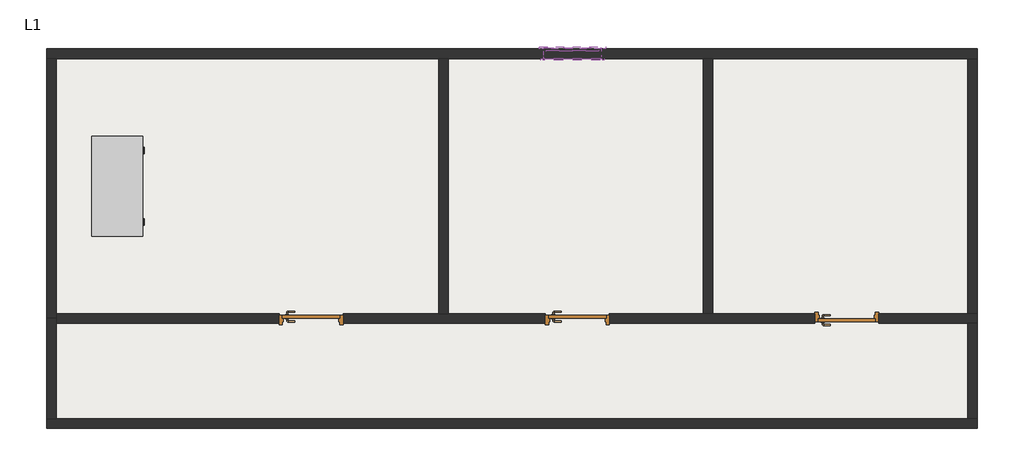
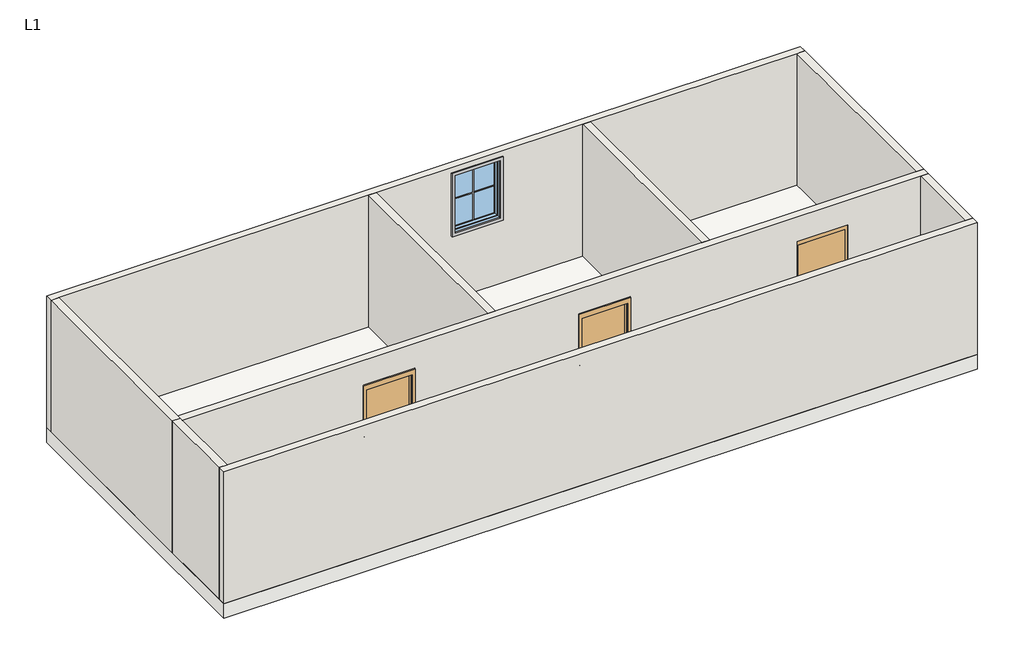
# One storey: 9 walls, 3 doors, 3 proxies, 1 furniture element, 1 slab, 1 window.
# Revit data of these elements (continued)
# Type "M_Muntin Pattern_2x2 : M_Muntin Pattern_2x2" (continued)
#   Width [instance default] = 1200 mm
#   Thickness = 12.7 mm
#   Height [instance default] = 1200 mm
#   Distance = 19.05 mm
#   Interior Material [instance default] = none
#   Exterior Material [instance default] = none
#   Default Elevation = 0
# Type "M_Trim-Window-Exterior-Flat : with Sill"
#   Trim Width = 60 mm
#   Trim Thickness_Picture Frame = 30 mm
#   Trim Thickness_with Sill = 19.05 mm
#   Sill Thickness = 30 mm
#   Opening Width [instance default] = 600 mm
#   Opening Height [instance default] = 900 mm
#   Default Elevation = 1200 mm
#   Sill = yes
#   Picture Frame = no
#   Trim Material [instance default] = none
# Type "M_Trim-Window-Interior-Flat : Picture Frame"
#   Trim Thickness_Picture Frame = 30 mm
#   Trim Width = 60 mm
#   Trim Thickness_with Sill = 20 mm
#   Sill Thickness = 30 mm
#   Opening Width [instance default] = 600 mm
#   Opening Height [instance default] = 900 mm
#   Default Elevation = 1200 mm
#   Sill = no
#   Picture Frame = yes
#   Trim Material [instance default] = none
# Type "M_Door-Passage-Single-Flush : 900 x 2100mm"
#   Type Mark = "38"
#   Analytic Construction = "Wooden"
#   Thickness = 45 mm
#   Thermal Resistance (R) = 0.455703 (m²·K)/W
#   Swing Angle [instance default] = 90.00°
#   Strike Height = 1000 mm
#   Rough Width [instance default] = 1000 mm
#   Rough Height [instance default] = 2200 mm
#   MF Opening Height [instance default] = 100 mm
#   MF Opening Width [instance default] = 100 mm
#   Inset Calculate [instance default] = 105 mm
#   Masonry Inset [instance default] = 25 mm
#   Height = 2100 mm
#   Width = 900 mm
#   Heat Transfer Coefficient (U) = 2.19465 W/(m²·K)
#   Masonry Frame Depth = 150 mm
#   Masonry Frame [instance default] = yes
#   Function = 1
#   Dry Wall Frame [instance default] = no
#   Panel Material = Wood - Birch
#   Frame Material = Metal - Paint Finish - Grey
#   Door Handle Material = Aluminum
#   Visual Light Transmittance = 0
#   Solar Heat Gain Coefficient = 0
#   Wall Closure = (empty or 0)
# Type "M_Desk : 1525 x 762mm Student"
#   Depth = 762 mm
#   Height = 762 mm
#   Leg Height = 152 mm
#   Width = 1525 mm
#   Body Material = Laminate, Ivory, Matte
#   Handle/Leg Material = Steel, Chrome Plated
#   Top Material = Cherry
#   Default Elevation = 0
# Type "Generic 300mm"
#   Description = "Generic Floor (Material By Category), 300mm thick"
#   Function = 0
#   Layers, outside or top first: 300 mm no material (function 1)
# Type "Generic - 150mm"
#   Description = "Generic Wall (Material By Category), 150mm thick"
#   Type Mark = "G04"
#   Layers, outside or top first: 150 mm no material (function 1)
# Type "M_Window-Fixed : 900 x 1200mm"
#   Type Mark = "36"
#   Fire Rating = "0.5h"
#   Analytic Construction = "Double glazing - domestic"
#   Window Inset [instance default] = 0 mm
#   Wall Thickness [instance default] = 150 mm
#   Visual Light Transmittance = 0.81
#   Thermal Resistance (R) = 0.319569 (m²·K)/W
#   Solar Heat Gain Coefficient = 0.76
#   Rough Width = 915 mm
#   Rough Height = 1215 mm
#   Interior Wall Closure [instance default] = 54.75 mm
#   Height = 1200 mm
#   Heat Transfer Coefficient (U) = 3.12929 W/(m²·K)
#   Frame Extension [instance default] = 6.35 mm
#   Exterior Wall Closure [instance default] = 31.75 mm
#   Extension Jamb [instance default] = 54.75 mm
#   Default Sill Height = 900 mm
#   Width = 900 mm
#   Muntin Visibility = yes
#   Interior Trim Visibility [instance default] = yes
#   Exterior Trim Visibility [instance default] = yes
#   Extension Jamb Visibility [instance default] = yes
#   Muntin Pattern = M_Muntin Pattern_2x2 : M_Muntin Pattern_2x2
#   Interior Trim Material = Wood - Stained
#   Interior Trim = M_Trim-Window-Interior-Flat : Picture Frame
#   Interior Frame Material = Wood - Stained
#   Glass Panel Material = Glass
#   Exterior Trim Material = Clad - White
#   Exterior Trim = M_Trim-Window-Exterior-Flat : with Sill
#   Exterior Frame Material = Clad - White
#   Wall Closure = (empty or 0)
# Element 1 (IfcBuildingElementProxy, "M_Muntin Pattern_2x2 : M_Muntin Pattern_2x2")
#   Width = 823.8 mm
#   Height = 1123.8 mm
#   Interior Material = Wood - Stained
#   Exterior Material = Clad - White
#   Phase Created = New Construction
#   Materials on its faces: "Clad - White", "Wood - Stained"
# Element 2 (IfcBuildingElementProxy, "M_Trim-Window-Exterior-Flat : with Sill")
#   Opening Width = 900 mm
#   Opening Height = 1200 mm
#   Trim Material = Clad - White
#   Phase Created = New Construction
#   Materials on its faces: "Clad - White"
# Element 3 (IfcBuildingElementProxy, "M_Trim-Window-Interior-Flat : Picture Frame")
#   Opening Width = 900 mm
#   Opening Height = 1200 mm
#   Trim Material = Wood - Stained
#   Phase Created = New Construction
#   Materials on its faces: "Wood - Stained"
# Elements 4, 5, 6 (IfcDoor, "M_Door-Passage-Single-Flush : 900 x 2100mm")
#   Swing Angle = 90.00°
#   Rough Width = 1000 mm
#   Rough Height = 2200 mm
#   Masonry Inset = 25 mm
#   MF Opening Width = 100 mm
#   MF Opening Height = 100 mm
#   Inset Calculate = 105 mm
#   Masonry Frame = yes
#   Dry Wall Frame = no
#   Phase Created = New Construction
#   Materials on its faces: "Aluminum", "Metal - Paint Finish - Grey", "Wood - Birch"
# Element 7 (IfcFurniture, "M_Desk : 1525 x 762mm Student")
#   Phase Created = New Construction
#   Materials on its faces: "Steel, Chrome Plated", "Laminate, Ivory, Matte", "Cherry"
# Element 8 (IfcSlab, "Generic 300mm")
#   Height Offset From Level = 0 mm
#   Phase Created = New Construction
#   Materials on its faces: "Default Floor"
# Elements 9, 10, 11, 12, 13, 14, 15, 17 (IfcWall, "Generic - 150mm")
#   Top Offset = 0 mm
#   Base Offset = 0 mm
#   Unconnected Height = 2700 mm
#   wall height = 2700 mm
#   Phase Created = New Construction
#   Base Constraint = L1
#   Materials on its faces: "Default Wall"
# Element 16 (IfcWall, "Generic - 150mm")
#   Top Offset = 0 mm
#   Base Offset = 0 mm
#   wall height = 2700 mm
#   Phase Created = New Construction
#   Base Constraint = L1
#   Top Constraint = L2
#   Materials on its faces: "Default Wall"
# Element 18 (IfcWindow, "M_Window-Fixed : 900 x 1200mm")
#   Mark = "107"
#   Window Inset = 0 mm
#   Interior Wall Closure = 54.75 mm
#   Frame Extension = 6.35 mm
#   Exterior Wall Closure = 31.75 mm
#   Interior Trim Visibility = yes
#   Exterior Trim Visibility = yes
#   Phase Created = New Construction
#   Materials on its faces: "Wood - Stained", "Glass", "Clad - White"
# Materials
#   "Wood - Birch": class "Wood", colour RGB 173 132 96, transparency 0, Cost = 0
#   "Metal - Paint Finish - Grey": class "Paint", colour RGB 178 178 178, transparency 0, Cost = 0
#   "Aluminum": class "Metal", colour RGB 244 245 246, transparency 0, Description = "Aluminum 6061", Cost = 0
#   "Laminate, Ivory, Matte": class "Plastic", colour RGB 244 244 244, transparency 0, Description = "Plastic Laminate - Ivory, Matte", Cost = 0
#   "Steel, Chrome Plated": class "Metal", colour RGB 17 17 17, transparency 0, Description = "Chromiuim plated steel", Cost = 0
#   "Cherry": class "Wood", colour RGB 158 77 40, transparency 0, Description = "Prunus Serotina", Cost = 0
#   "Wood - Stained": class "Wood", colour RGB 173 132 96, transparency 0, Cost = 0
#   "Glass": class "Glass", colour RGB 245 245 243, transparency 1, Description = "Soda Lime Glass", Cost = 0
#   "Clad - White": class "Wood", colour RGB 245 245 243, transparency 0, Cost = 0
#   "Default Floor": class "Miscellaneous", colour RGB 128 128 128, transparency 0, Cost = 0
#   "Default Wall": class "Miscellaneous", colour RGB 192 192 192, transparency 0, Cost = 0
# Room at (6067.793, 2177.027) mm, phase "New Construction", upper level "L1", upper offset 3048 mm, lower offset 0 mm
#   Number = "100"
#   Name = "Room Name"
# Room at (1924.302, 2177.027) mm, phase "New Construction", upper level "L1", upper offset 3048 mm, lower offset 0 mm
#   Number = "101"
#   Name = "Room Name"
# Room at (-2925.467, 2177.027) mm, phase "New Construction", upper level "L1", upper offset 3048 mm, lower offset 0 mm
#   Number = "102"
#   Name = "Room Name"
# Room at (1500.535, -930.592) mm, phase "New Construction", upper level "L1", upper offset 3048 mm, lower offset 0 mm
#   Number = "103"
#   Name = "Room Name"
